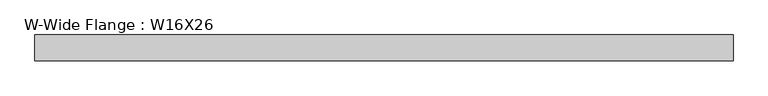
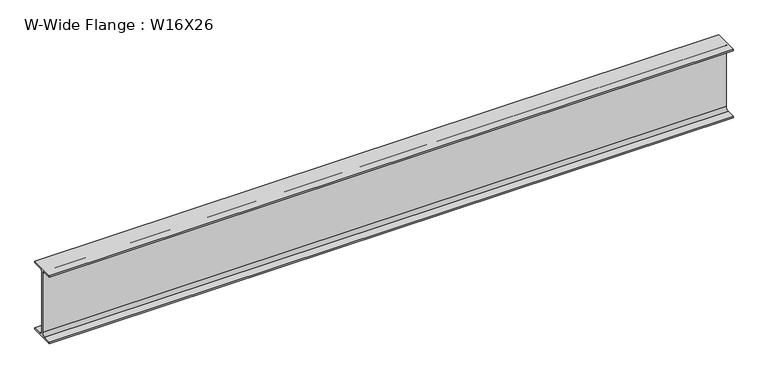
"""IFC4 building model written with IfcOpenShell, lengths in millimetres: beam geometry, W-Wide Flange : W16X26."""

from ifc_helpers import new_model, si_unit, point, frame, frame_2d, origin, place, context, project, spatial, polyline, circle_curve, trimmed, segment, composite_curve, outline, extrude, source, transform, mapped, element, save


def w_wide_flange_w16x26_702b2a89(model_context):
    return source(origin(), model_context, "Body", "SweptSolid", [
        extrude(outline(composite_curve([segment(polyline([(69.85, -190.627), (69.85, -199.39), (-69.85, -199.39), (-69.85, -190.627), (-21.3995, -190.627)]), True, "CONTINUOUS"), segment(trimmed(circle_curve(frame_2d((-21.3995, -172.4025)), 18.2245), [point((-21.3995, -190.627))], [point((-3.175, -172.4025))], True, "CARTESIAN"), True, "CONTINUOUS"), segment(polyline([(-3.175, -172.4025), (-3.175, 172.4025)]), True, "CONTINUOUS"), segment(trimmed(circle_curve(frame_2d((-21.3995, 172.4025)), 18.2245), [point((-3.175, 172.4025))], [point((-21.3995, 190.627))], True, "CARTESIAN"), True, "CONTINUOUS"), segment(polyline([(-21.3995, 190.627), (-69.85, 190.627), (-69.85, 199.39), (69.85, 199.39), (69.85, 190.627), (21.3995, 190.627)]), True, "CONTINUOUS"), segment(trimmed(circle_curve(frame_2d((21.3995, 172.4025)), 18.2245), [point((21.3995, 190.627))], [point((3.175, 172.4025))], True, "CARTESIAN"), True, "CONTINUOUS"), segment(polyline([(3.175, 172.4025), (3.175, -172.4025)]), True, "CONTINUOUS"), segment(trimmed(circle_curve(frame_2d((21.3995, -172.4025)), 18.2245), [point((3.175, -172.4025))], [point((21.3995, -190.627))], True, "CARTESIAN"), True, "CONTINUOUS"), segment(polyline([(21.3995, -190.627), (69.85, -190.627)]), True, "CONTINUOUS")], self_intersect=False)), frame((-1892.3, 0.0, 0.0), z_axis=(1.0, 0.0, 0.0), x_axis=(0.0, 1.0, 0.0)), (0.0, 0.0, 1.0), 3784.346),
    ])


if __name__ == "__main__":
    model = new_model("IFC4")
    model_context = context("Model", 3, world=origin())
    ifc_project = project(units=[si_unit("LENGTHUNIT", "METRE", prefix="MILLI")], contexts=[model_context])
    site = spatial("IfcSite", under=ifc_project)
    building = spatial("IfcBuilding", under=site)
    placement = place(None, origin())
    w_wide_flange_w16x26_shape = w_wide_flange_w16x26_702b2a89(model_context)
    element("IfcBeam", 1, ObjectType="W-Wide Flange : W16X26", at=placement, inside=building, context=model_context, shape_type="MappedRepresentation", body=[
        mapped(w_wide_flange_w16x26_shape, transform((0.0, 0.0, 0.0), x_axis=(1.0, 0.0, 0.0), y_axis=(0.0, 1.0, 0.0), z_axis=(0.0, 0.0, 1.0))),
    ])
    save(model, "model.ifc")

# Revit data of these elements
# Type "W-Wide Flange : W16X26"
#   Assembly Code = "B10"
#   W = 26
#   Length [instance default] = 5' - 0"
#   bf = 0' - 5 1/2"
#   d = 1' - 3.7"
#   k = 0' - 1 1/16"
#   k2 = 0' - 0.7175"
#   tf = 0' - 0.345"
#   tw = 0' - 0 1/4"
#   A = 0.0533333 SF
#   Structural Material [instance default] = Steel ASTM A992
# Element 1 (IfcBeam, "W-Wide Flange : W16X26")
#   Materials on its faces: "Steel ASTM A992"
# Materials
#   "Steel ASTM A992": class "Metal", colour RGB 199 199 199, transparency 0, Description = "Structural steel 50ksi", Cost = 0
